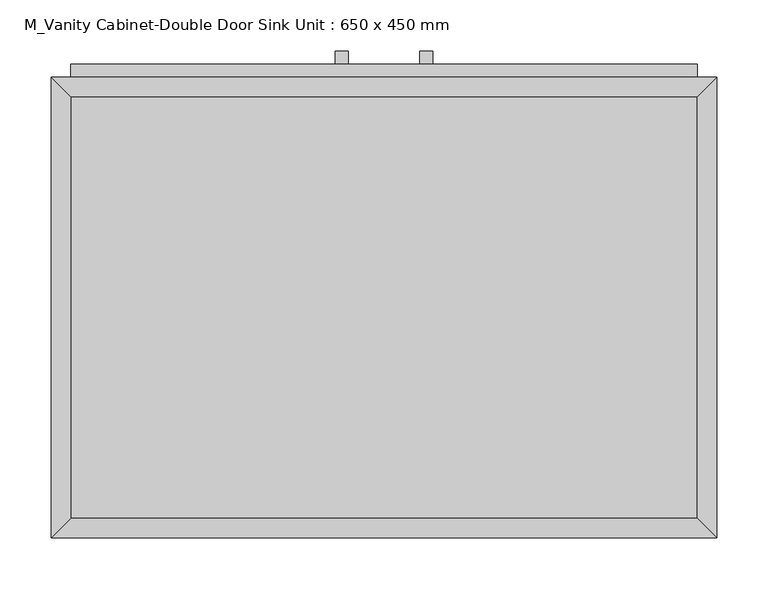
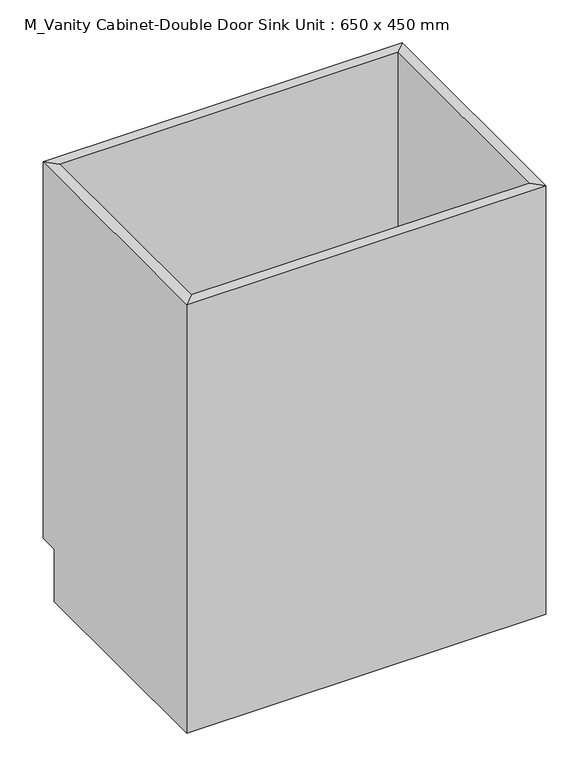
"""IFC4 building model written with IfcOpenShell, lengths in millimetres: furniture geometry, M_Vanity Cabinet-Double Door Sink Unit : 650 x 450 mm."""

from ifc_helpers import new_model, si_unit, frame, origin, place, context, project, spatial, polyline, outline, extrude, faceted_brep, source, transform, mapped, element, save


def m_vanity_cabinet_double_door_sink_unit_650_x_450_mm_18d6df3f(model_context):
    return source(origin(), model_context, "Body", "SolidModel", [
        faceted_brep([(324.6877049, 430.95, 820.0), (-287.2122951, 430.95, 820.0), (-287.2122951, 430.95, 100.0), (324.6877049, 430.95, 100.0), (343.7377049, 450.0, 820.0), (-306.2622951, 450.0, 820.0), (343.7377049, 450.0, 100.0), (-306.2622951, 450.0, 100.0), (-287.2122951, 19.05, 820.0), (-287.2122951, 19.05, 100.0), (-287.2122951, 415.0, 100.0), (-306.2622951, 0.0, 820.0), (-306.2622951, 415.0, 100.0), (-306.2622951, 415.0, 0.0), (-306.2622951, 0.0, 0.0), (324.6877049, 19.05, 820.0), (324.6877049, 19.05, 100.0), (343.7377049, 0.0, 820.0), (343.7377049, 0.0, 0.0), (324.6877049, 415.0, 100.0), (343.7377049, 415.0, 0.0), (343.7377049, 415.0, 100.0)], [[[0, 1, 2, 3]], [[0, 4, 5, 1]], [[4, 6, 7, 5]], [[2, 7, 6, 3]], [[1, 8, 9, 10, 2]], [[5, 11, 8, 1]], [[7, 12, 13, 14, 11, 5]], [[2, 10, 12, 7]], [[8, 15, 16, 9]], [[11, 17, 15, 8]], [[14, 18, 17, 11]], [[3, 19, 16, 15, 0]], [[0, 15, 17, 4]], [[4, 17, 18, 20, 21, 6]], [[6, 21, 19, 3]], [[10, 9, 16, 19]], [[18, 14, 13, 20]], [[13, 12, 10, 19, 21, 20]]]),
        extrude(outline(polyline([(-16.1872951, 475.4), (-16.1872951, 462.7), (-28.8872951, 462.7), (-28.8872951, 475.4), (-16.1872951, 475.4)])), frame((0.0, 0.0, 517.469895), z_axis=(0.0, 0.0, 1.0), x_axis=(1.0, 0.0, 0.0)), (0.0, 0.0, 1.0), 124.730105),
        extrude(outline(polyline([(66.3627049, 475.4), (66.3627049, 462.7), (53.6627049, 462.7), (53.6627049, 475.4), (66.3627049, 475.4)])), frame((0.0, 0.0, 517.469895), z_axis=(0.0, 0.0, 1.0), x_axis=(1.0, 0.0, 0.0)), (0.0, 0.0, 1.0), 124.730105),
        extrude(outline(polyline([(9.2127049, 462.7), (9.2127049, 450.0), (-287.2122951, 450.0), (-287.2122951, 462.7), (9.2127049, 462.7)])), frame((0.0, 0.0, 119.05), z_axis=(0.0, 0.0, 1.0), x_axis=(1.0, 0.0, 0.0)), (0.0, 0.0, 1.0), 561.25),
        extrude(outline(polyline([(324.6877049, 462.7), (324.6877049, 450.0), (28.2627049, 450.0), (28.2627049, 462.7), (324.6877049, 462.7)])), frame((0.0, 0.0, 119.05), z_axis=(0.0, 0.0, 1.0), x_axis=(1.0, 0.0, 0.0)), (0.0, 0.0, 1.0), 561.25),
        extrude(outline(polyline([(324.6877049, 462.7), (324.6877049, 450.0), (-287.2122951, 450.0), (-287.2122951, 462.7), (324.6877049, 462.7)])), frame((0.0, 0.0, 699.35), z_axis=(0.0, 0.0, 1.0), x_axis=(1.0, 0.0, 0.0)), (0.0, 0.0, 1.0), 101.6),
        extrude(outline(polyline([(324.6877049, 19.05), (-287.2122951, 19.05), (-287.2122951, 430.95), (324.6877049, 430.95), (324.6877049, 19.05)])), frame((0.0, 0.0, 100.0), z_axis=(0.0, 0.0, 1.0), x_axis=(1.0, 0.0, 0.0)), (0.0, 0.0, 1.0), 19.05),
    ])


if __name__ == "__main__":
    model = new_model("IFC4")
    model_context = context("Model", 3, world=origin())
    ifc_project = project(units=[si_unit("LENGTHUNIT", "METRE", prefix="MILLI")], contexts=[model_context])
    site = spatial("IfcSite", under=ifc_project)
    building = spatial("IfcBuilding", under=site)
    placement = place(None, origin())
    m_vanity_cabinet_double_door_sink_unit_650_x_450_mm_shape = m_vanity_cabinet_double_door_sink_unit_650_x_450_mm_18d6df3f(model_context)
    element("IfcFurniture", 1, ObjectType="M_Vanity Cabinet-Double Door Sink Unit : 650 x 450 mm", at=placement, inside=building, context=model_context, shape_type="MappedRepresentation", body=[
        mapped(m_vanity_cabinet_double_door_sink_unit_650_x_450_mm_shape, transform((0.0, 0.0, 0.0), x_axis=(1.0, 0.0, 0.0), y_axis=(0.0, 1.0, 0.0), z_axis=(0.0, 0.0, 1.0))),
    ])
    save(model, "model.ifc")

# Revit data of these elements
# Type "M_Vanity Cabinet-Double Door Sink Unit : 650 x 450 mm"
#   Manufacturer = "Manufacturer"
#   Finish = "Finish"
#   Construction Type = "Construction Type"
#   AccessibilityPerformance = "AccessibilityPerformance"
#   CodePerformance = "CodePerformance"
#   Area = "Area"
#   Color = "Color"
#   Constituents = "Constituents"
#   Features = "Features"
#   Finish = "Finish"
#   Grade = "Grade"
#   Material = "Material"
#   ModelReference = "ModelReference"
#   NominalHeight = "NominalHeight"
#   NominalLength = "NominalLength"
#   NominalWidth = "NominalWidth"
#   ProductionYear = "ProductionYear"
#   Reference = "Reference"
#   Shape = "Shape"
#   Size = "Size"
#   SustainabilityPerformance = "SustainabilityPerformance"
#   WarrantyDescription = "WarrantyDescription"
#   WarrantyDurationLabor = "WarrantyDurationLabor"
#   WarrantyDurationParts = "WarrantyDurationParts"
#   WarrantyGuarantorLabor = "WarrantyGuarantorLabor"
#   WarrantyGuarantorParts = "WarrantyGuarantorParts"
#   ExpectedLife = "ExpectedLife"
#   ReplacementCost = "ReplacementCost"
#   AssetAccountingType = "FIXED"
#   ModelLabel = "ModelLabel"
#   Depth = 0.450 m
#   Height = 0.820 m
#   Plinth Depth = 0.035 m
#   Plinth Height = 0.100 m
#   Width = 0.650 m
#   Cabinet Material = none
#   Door/Drawer Material = none
#   Handle Material = Cabinets - Handles
# Element 1 (IfcFurniture, "M_Vanity Cabinet-Double Door Sink Unit : 650 x 450 mm")
#   Materials on its faces: "Cabinets", "Cabinets - Handles"
# Materials
#   "Cabinets - Handles": class "Metal", colour RGB 57 57 57, transparency 0
#   "Cabinets": class "Miscellaneous", colour RGB 249 249 249, transparency 0
